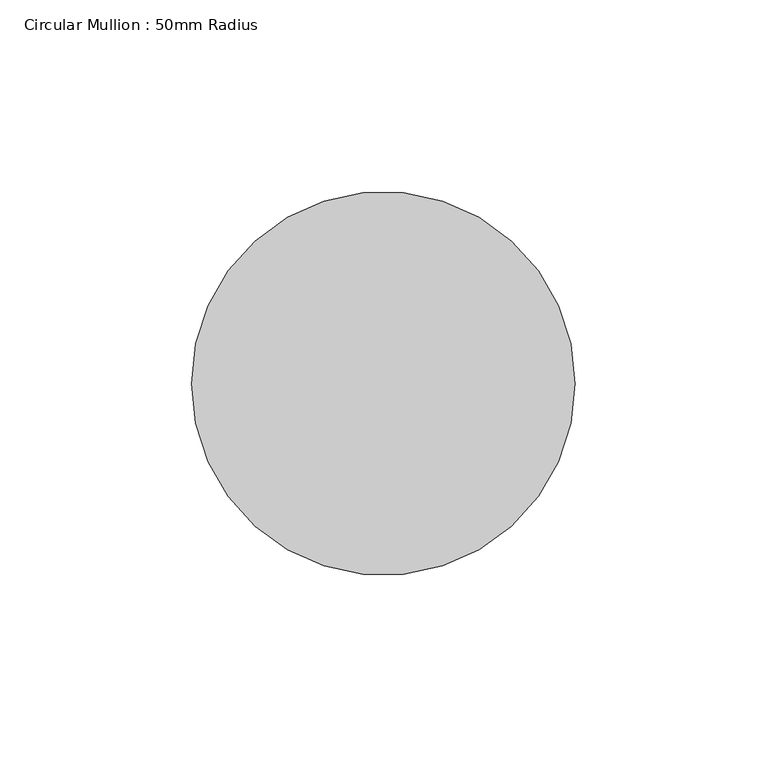
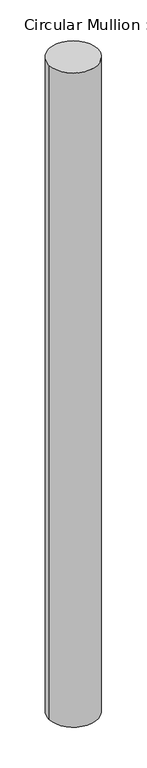
"""IFC4 building model written with IfcOpenShell, lengths in millimetres: member geometry, Circular Mullion : 50mm Radius."""

from ifc_helpers import new_model, si_unit, point, frame, origin, origin_2d, place, context, project, spatial, circle_curve, trimmed, segment, composite_curve, outline, extrude, source, transform, mapped, element, save


def circular_mullion_50mm_radius_292e4b68(model_context):
    return source(origin(), model_context, "Body", "SweptSolid", [
        extrude(outline(composite_curve([segment(trimmed(circle_curve(origin_2d(), 50.0), [point((50.0, 0.0))], [point((-50.0, 0.0))], False, "CARTESIAN"), True, "CONTINUOUS"), segment(trimmed(circle_curve(origin_2d(), 50.0), [point((-50.0, 0.0))], [point((50.0, 0.0))], False, "CARTESIAN"), True, "CONTINUOUS")], self_intersect=False)), frame((0.0, 0.0, -1420.074279), z_axis=(0.0, 0.0, 1.0), x_axis=(1.0, 0.0, 0.0)), (0.0, 0.0, 1.0), 1420.074279),
    ])


if __name__ == "__main__":
    model = new_model("IFC4")
    model_context = context("Model", 3, world=origin())
    ifc_project = project(units=[si_unit("LENGTHUNIT", "METRE", prefix="MILLI")], contexts=[model_context])
    site = spatial("IfcSite", under=ifc_project)
    building = spatial("IfcBuilding", under=site)
    placement = place(None, origin())
    circular_mullion_50mm_radius_shape = circular_mullion_50mm_radius_292e4b68(model_context)
    element("IfcMember", 1, ObjectType="Circular Mullion : 50mm Radius", at=placement, inside=building, context=model_context, shape_type="MappedRepresentation", body=[
        mapped(circular_mullion_50mm_radius_shape, transform((0.0, 0.0, 0.0), x_axis=(1.0, 0.0, 0.0), y_axis=(0.0, 1.0, 0.0), z_axis=(0.0, 0.0, 1.0))),
    ])
    save(model, "model.ifc")

# Revit data of these elements
# Type "Circular Mullion : 50mm Radius"
#   built-in parameter 1007350 = 0.164042 (stored number, unit not read)
# Element 1 (IfcMember, "Circular Mullion : 50mm Radius")
#   Materials on its faces: "Aluminium"
# Materials
#   "Aluminium": class "Metal", colour RGB 247 247 247, transparency 0, Description = "Aluminium 6061", Cost = 0
